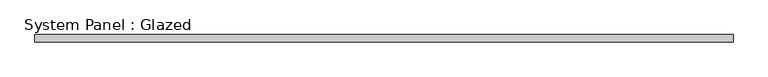
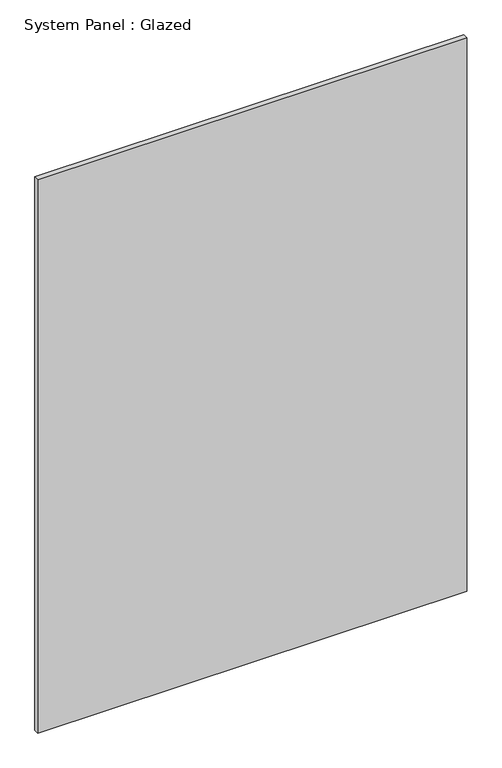
"""IFC4 building model written with IfcOpenShell, lengths in millimetres: plate geometry, System Panel : Glazed."""

from ifc_helpers import new_model, si_unit, origin, origin_with_axes, place, context, project, spatial, polyline, outline, extrude, source, transform, mapped, element, save


def system_panel_glazed_4b2262bb(model_context):
    return source(origin(), model_context, "Body", "SweptSolid", [
        extrude(outline(polyline([(1162.2216647, 24.5), (-1162.2216647, 24.5), (-1162.2216647, 49.5), (1162.2216647, 49.5), (1162.2216647, 24.5)])), origin_with_axes(), (0.0, 0.0, 1.0), 3170.0),
    ])


if __name__ == "__main__":
    model = new_model("IFC4")
    model_context = context("Model", 3, world=origin())
    ifc_project = project(units=[si_unit("LENGTHUNIT", "METRE", prefix="MILLI")], contexts=[model_context])
    site = spatial("IfcSite", under=ifc_project)
    building = spatial("IfcBuilding", under=site)
    placement = place(None, origin())
    system_panel_glazed_shape = system_panel_glazed_4b2262bb(model_context)
    element("IfcPlate", 1, ObjectType="System Panel : Glazed", at=placement, inside=building, context=model_context, shape_type="MappedRepresentation", body=[
        mapped(system_panel_glazed_shape, transform((0.0, 0.0, 0.0), x_axis=(1.0, 0.0, 0.0), y_axis=(0.0, 1.0, 0.0), z_axis=(0.0, 0.0, 1.0))),
    ])
    save(model, "model.ifc")

# Revit data of these elements
# Type "System Panel : Glazed"
#   Construction Type Id = "GSP4R"
#   Analytic Construction = "1/8 in Pilkington single glazing"
#   Visual Light Transmittance = 0.9
#   Solar Heat Gain Coefficient = 0.86
#   Heat Transfer Coefficient (U) = 6.7069 W/(m²·K)
#   Define Thermal Properties by = 1
# Element 1 (IfcPlate, "System Panel : Glazed")
#   Materials on its faces: "Glass"
# Materials
#   "Glass": class "Glass", colour RGB 245 245 243, transparency 1, Description = "Soda Lime Glass", Cost = 0
